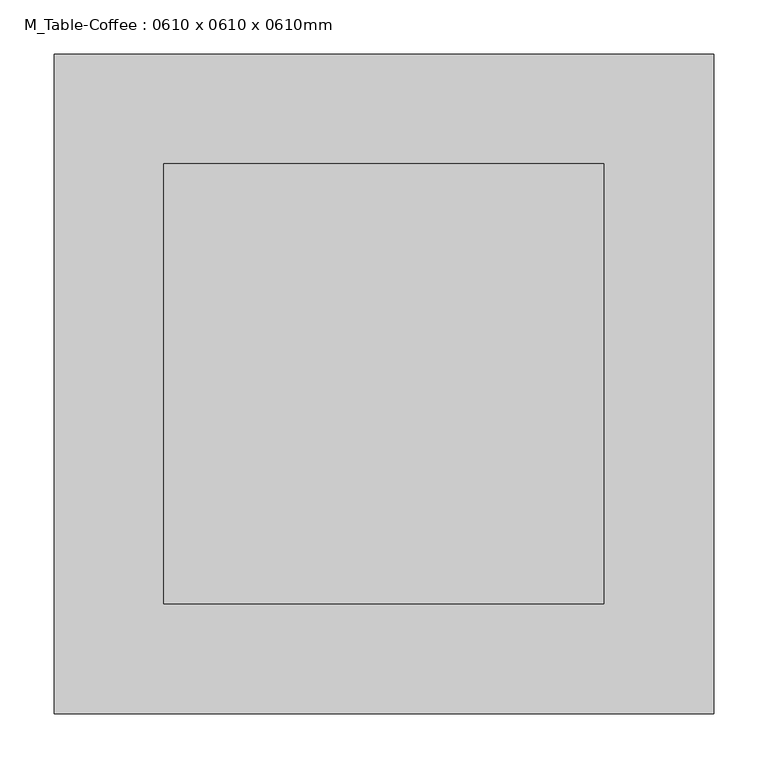
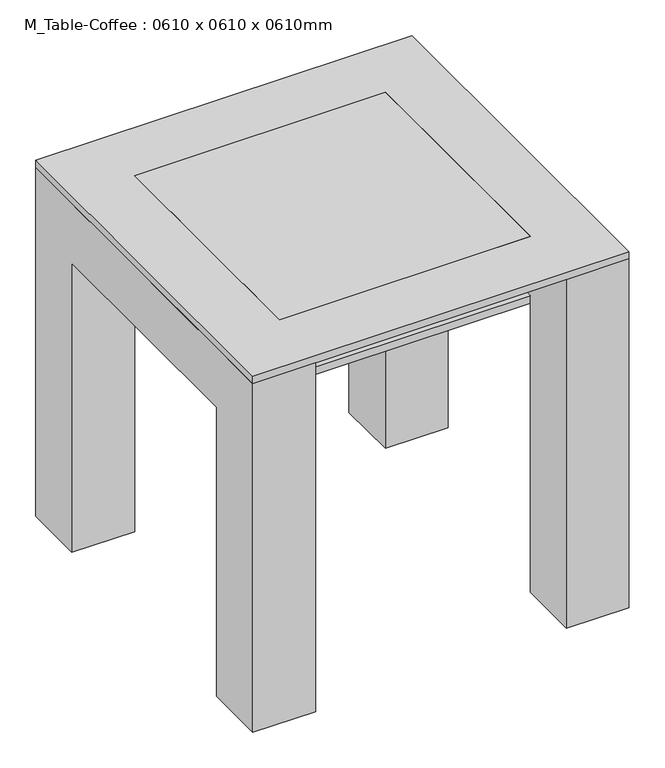
"""IFC4 building model written with IfcOpenShell, lengths in millimetres: furniture geometry, M_Table-Coffee : 0610 x 0610 x 0610mm."""

from ifc_helpers import new_model, si_unit, frame, origin, place, context, project, spatial, polyline, outline, extrude, source, transform, mapped, element, save


def m_table_coffee_0610_x_0610_x_0610mm_65ce43c2(model_context):
    return source(origin(), model_context, "Body", "SweptSolid", [
        extrude(outline(polyline([(221.6657667, 298.6110778), (221.6657667, -108.1889222), (-185.1342333, -108.1889222), (-185.1342333, 298.6110778), (221.6657667, 298.6110778)])), frame((0.0, 0.0, 495.7), z_axis=(0.0, 0.0, 1.0), x_axis=(1.0, 0.0, 0.0)), (0.0, 0.0, 1.0), 12.7),
        extrude(outline(polyline([(400.2110778, 0.0), (298.6110778, 0.0), (298.6110778, 495.7), (-108.1889222, 495.7), (-108.1889222, 0.0), (-209.7889222, 0.0), (-209.7889222, 597.3), (400.2110778, 597.3), (400.2110778, 0.0)])), frame((221.6657667, 0.0, 0.0), z_axis=(1.0, 0.0, 0.0), x_axis=(0.0, 1.0, 0.0)), (0.0, 0.0, 1.0), 101.6),
        extrude(outline(polyline([(400.2110778, 597.3), (400.2110778, 0.0), (298.6110778, 0.0), (298.6110778, 495.7), (-108.1889222, 495.7), (-108.1889222, 0.0), (-209.7889222, 0.0), (-209.7889222, 597.3), (400.2110778, 597.3)])), frame((-286.7342333, 0.0, 0.0), z_axis=(1.0, 0.0, 0.0), x_axis=(0.0, 1.0, 0.0)), (0.0, 0.0, 1.0), 101.6),
        extrude(outline(polyline([(221.6657667, 298.6110778), (221.6657667, -108.1889222), (-185.1342333, -108.1889222), (-185.1342333, 298.6110778), (221.6657667, 298.6110778)])), frame((0.0, 0.0, 597.3), z_axis=(0.0, 0.0, 1.0), x_axis=(1.0, 0.0, 0.0)), (0.0, 0.0, 1.0), 12.7),
        extrude(outline(polyline([(323.2657667, 400.2110778), (323.2657667, -209.7889222), (-286.7342333, -209.7889222), (-286.7342333, 400.2110778), (323.2657667, 400.2110778)]), holes=[polyline([(221.6657667, 298.6110778), (-185.1342333, 298.6110778), (-185.1342333, -108.1889222), (221.6657667, -108.1889222), (221.6657667, 298.6110778)])]), frame((0.0, 0.0, 597.3), z_axis=(0.0, 0.0, 1.0), x_axis=(1.0, 0.0, 0.0)), (0.0, 0.0, 1.0), 12.7),
    ])


if __name__ == "__main__":
    model = new_model("IFC4")
    model_context = context("Model", 3, world=origin())
    ifc_project = project(units=[si_unit("LENGTHUNIT", "METRE", prefix="MILLI")], contexts=[model_context])
    site = spatial("IfcSite", under=ifc_project)
    building = spatial("IfcBuilding", under=site)
    placement = place(None, origin())
    m_table_coffee_0610_x_0610_x_0610mm_shape = m_table_coffee_0610_x_0610_x_0610mm_65ce43c2(model_context)
    element("IfcFurniture", 1, ObjectType="M_Table-Coffee : 0610 x 0610 x 0610mm", at=placement, inside=building, context=model_context, shape_type="MappedRepresentation", body=[
        mapped(m_table_coffee_0610_x_0610_x_0610mm_shape, transform((0.0, 0.0, 0.0), x_axis=(1.0, 0.0, 0.0), y_axis=(0.0, 1.0, 0.0), z_axis=(0.0, 0.0, 1.0))),
    ])
    save(model, "model.ifc")

# Revit data of these elements
# Type "M_Table-Coffee : 0610 x 0610 x 0610mm"
#   Manufacturer = "Manufacturer"
#   AccessibilityPerformance = "AccessibilityPerformance"
#   CodePerformance = "CodePerformance"
#   Area = "Area"
#   Color = "Color"
#   Constituents = "Constituents"
#   Features = "Features"
#   Finish = "Finish"
#   Grade = "Grade"
#   Material = "Material"
#   ModelReference = "ModelReference"
#   NominalHeight = "NominalHeight"
#   NominalLength = "NominalLength"
#   NominalWidth = "NominalWidth"
#   ProductionYear = "ProductionYear"
#   Reference = "Reference"
#   Shape = "Shape"
#   Size = "Size"
#   SustainabilityPerformance = "SustainabilityPerformance"
#   WarrantyDescription = "WarrantyDescription"
#   WarrantyDurationLabor = "WarrantyDurationLabor"
#   WarrantyDurationParts = "WarrantyDurationParts"
#   WarrantyGuarantorLabor = "WarrantyGuarantorLabor"
#   WarrantyGuarantorParts = "WarrantyGuarantorParts"
#   ExpectedLife = "ExpectedLife"
#   ReplacementCost = "ReplacementCost"
#   AssetAccountingType = "NONFIXED"
#   ModelLabel = "ModelLabel"
#   Height = 0.610 m
#   Length = 0.610 m
#   Width = 0.610 m
#   Top Material = Metal - Chrome
#   Frame Material = Wood - Teak
# Element 1 (IfcFurniture, "M_Table-Coffee : 0610 x 0610 x 0610mm")
#   Materials on its faces: "Wood - Teak", "Metal - Chrome", "Glass - Clear, Grey"
# Materials
#   "Metal - Chrome": class "Metal", colour RGB 17 17 17, transparency 0
#   "Wood - Teak": class "Wood", colour RGB 145 112 90, transparency 0
#   "Glass - Clear, Grey": class "Glass", colour RGB 252 255 255, transparency 0.64
